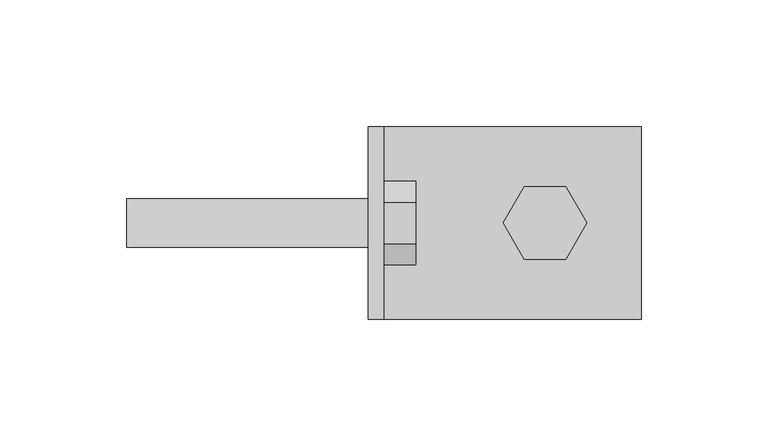
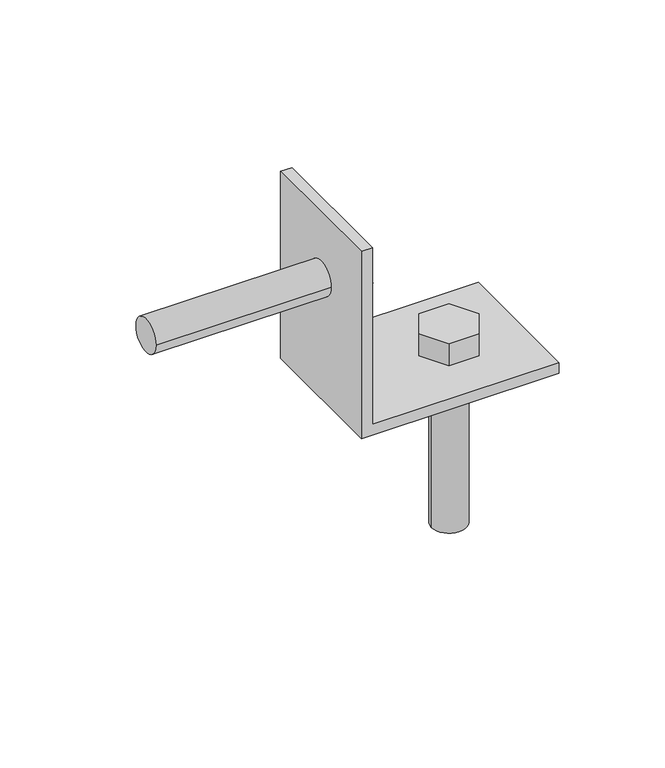
"""IFC4 building model written with IfcOpenShell, lengths in millimetres: fastener geometry, SIMPSON - HLPC/HLGPC Heavy Angles and Gussets : SIMPSON - HL43 - 3 X 4.25 - .75 Bolt - HDG."""

import ifcopenshell
import ifcopenshell.guid

model = None  # the IFC model being written
_history = None  # IfcOwnerHistory: only IFC2X3 demands one
_inside = {}  # id of a spatial element -> (the spatial element, [elements in it])
_under = {}  # id of a project, library or spatial element -> (it, [spatial elements below it])
_declared = {}  # id of a project -> (the project, [libraries it declares])
_typed = {}  # id of a type object -> (the type object, [elements of that type])
_made_of = {}  # id of a material, layer set ... -> (it, [elements and type objects made of it])


def new_model(schema):
    """Start an empty IFC model of exactly this schema.

    Asked for "IFC4X3", IfcOpenShell would pick the latest addendum, in which some entities
    have other attributes; the version numbers below select the first issue.
    IFC2X3 requires an IfcOwnerHistory on every rooted entity: one is made here for all.
    """
    global model, _history
    if schema == "IFC4X3":
        model = ifcopenshell.file(schema_version=(4, 3, 0, 0))
    else:
        model = ifcopenshell.file(schema=schema)
    _inside.clear()
    _under.clear()
    _declared.clear()
    _typed.clear()
    _made_of.clear()
    _history = None
    if model.schema == "IFC2X3":
        org = make("IfcOrganization", Name="unknown")
        user = make(
            "IfcPersonAndOrganization",
            ThePerson=make("IfcPerson", FamilyName="unknown"),
            TheOrganization=org,
        )
        app = make(
            "IfcApplication",
            ApplicationDeveloper=org,
            Version="unknown",
            ApplicationFullName="unknown",
            ApplicationIdentifier="unknown",
        )
        _history = make(
            "IfcOwnerHistory",
            OwningUser=user,
            OwningApplication=app,
            ChangeAction="ADDED",
            CreationDate=0,
        )
    return model


def make(cls, **values):
    """One entity of the class cls with the attributes given. An attribute that is None is left unset."""
    return model.create_entity(
        cls, **{name: value for name, value in values.items() if value is not None}
    )


def rooted(cls, **values):
    """An entity with a GlobalId (a new one), such as an element, a storey or a relation."""
    return make(cls, GlobalId=ifcopenshell.guid.new(), OwnerHistory=_history, **values)


def si_unit(unit_type, name, prefix=None):
    """IfcSIUnit, for example si_unit("LENGTHUNIT", "METRE", prefix="MILLI")."""
    return make("IfcSIUnit", UnitType=unit_type, Prefix=prefix, Name=name)


def assignment(units):
    """IfcUnitAssignment: the units of a project."""
    return None if units is None else make("IfcUnitAssignment", Units=units)


def point(xyz):
    """IfcCartesianPoint."""
    return None if xyz is None else make("IfcCartesianPoint", Coordinates=xyz)


def direction(xyz):
    """IfcDirection."""
    return None if xyz is None else make("IfcDirection", DirectionRatios=xyz)


def frame(location, z_axis=None, x_axis=None):
    """IfcAxis2Placement3D, a coordinate frame: its origin and axes. An axis left out is left unset."""
    return make(
        "IfcAxis2Placement3D",
        Location=point(location),
        Axis=direction(z_axis),
        RefDirection=direction(x_axis),
    )


def frame_2d(location, x_axis=None):
    """IfcAxis2Placement2D, a coordinate frame in the plane: its origin and x axis."""
    return make(
        "IfcAxis2Placement2D", Location=point(location), RefDirection=direction(x_axis)
    )


def origin():
    """The frame at (0, 0, 0) with its axes left unset."""
    return frame((0.0, 0.0, 0.0))


def place(relative_to, where):
    """IfcLocalPlacement: puts the frame where relative to a parent placement (None: the world)."""
    return make(
        "IfcLocalPlacement", PlacementRelTo=relative_to, RelativePlacement=where
    )


def context(
    kind, dimensions, precision=None, world=None, true_north=None, identifier=None
):
    """IfcGeometricRepresentationContext, for example the 3D "Model" context."""
    return make(
        "IfcGeometricRepresentationContext",
        ContextIdentifier=identifier,
        ContextType=kind,
        CoordinateSpaceDimension=dimensions,
        Precision=precision,
        WorldCoordinateSystem=world,
        TrueNorth=true_north,
    )


def project(units=None, contexts=None):
    """IfcProject with its units and contexts."""
    return rooted(
        "IfcProject",
        Name="project",
        RepresentationContexts=contexts,
        UnitsInContext=assignment(units),
    )


def spatial(cls, under=None, at=None, **own):
    """A site, building, storey or space (cls), placed at a placement, below another one or the project."""
    s = rooted(cls, ObjectPlacement=at, **own)
    if under is not None:
        _under.setdefault(under.id(), (under, []))[1].append(s)
    return s


def polyline(points):
    """IfcPolyline through the points."""
    return make("IfcPolyline", Points=[point(p) for p in points])


def circle_curve(where, radius):
    """IfcCircle in the frame where."""
    return make("IfcCircle", Position=where, Radius=radius)


def trimmed(basis, trim1, trim2, sense, master):
    """IfcTrimmedCurve: the piece of a basis curve between two trims."""
    return make(
        "IfcTrimmedCurve",
        BasisCurve=basis,
        Trim1=trim1,
        Trim2=trim2,
        SenseAgreement=sense,
        MasterRepresentation=master,
    )


def segment(curve, same_sense, transition):
    """IfcCompositeCurveSegment."""
    return make(
        "IfcCompositeCurveSegment",
        Transition=transition,
        SameSense=same_sense,
        ParentCurve=curve,
    )


def composite_curve(segments, self_intersect=None):
    """IfcCompositeCurve: segments joined end to end."""
    return make("IfcCompositeCurve", Segments=segments, SelfIntersect=self_intersect)


def outline(outer, holes=None, kind="AREA"):
    """IfcArbitraryClosedProfileDef: a profile drawn as a closed curve; with holes, ...WithVoids."""
    if holes is None:
        return make("IfcArbitraryClosedProfileDef", ProfileType=kind, OuterCurve=outer)
    return make(
        "IfcArbitraryProfileDefWithVoids",
        ProfileType=kind,
        OuterCurve=outer,
        InnerCurves=holes,
    )


def extrude(swept, where, along, depth):
    """IfcExtrudedAreaSolid: the profile swept, set in the frame where, extruded along a direction by depth."""
    return make(
        "IfcExtrudedAreaSolid",
        SweptArea=swept,
        Position=where,
        ExtrudedDirection=direction(along),
        Depth=depth,
    )


def shape(context_of_items, identifier, shape_type, items):
    """IfcShapeRepresentation: the items that make up one representation, for example the "Body"."""
    return make(
        "IfcShapeRepresentation",
        ContextOfItems=context_of_items,
        RepresentationIdentifier=identifier,
        RepresentationType=shape_type,
        Items=items,
    )


def source(mapping_origin, context_of_items, identifier, shape_type, items):
    """IfcRepresentationMap: a shape defined once, which mapped items show again and again."""
    return make(
        "IfcRepresentationMap",
        MappingOrigin=mapping_origin,
        MappedRepresentation=shape(context_of_items, identifier, shape_type, items),
    )


def transform(
    local_origin,
    x_axis=None,
    y_axis=None,
    z_axis=None,
    scale=None,
    scale2=None,
    scale3=None,
    uniform=True,
):
    """IfcCartesianTransformationOperator3D, or its non-uniform kind. x_axis, y_axis, z_axis: its Axis1, 2, 3."""
    if uniform:
        return make(
            "IfcCartesianTransformationOperator3D",
            Axis1=direction(x_axis),
            Axis2=direction(y_axis),
            LocalOrigin=point(local_origin),
            Scale=scale,
            Axis3=direction(z_axis),
        )
    return make(
        "IfcCartesianTransformationOperator3DnonUniform",
        Axis1=direction(x_axis),
        Axis2=direction(y_axis),
        LocalOrigin=point(local_origin),
        Scale=scale,
        Axis3=direction(z_axis),
        Scale2=scale2,
        Scale3=scale3,
    )


def mapped(mapping_source, mapping_target):
    """IfcMappedItem: shows the shape of a source again, moved by a transform."""
    return make(
        "IfcMappedItem", MappingSource=mapping_source, MappingTarget=mapping_target
    )


def made_of(thing, what):
    """Note that an element or type object is made of a material, layer set ...; save() writes the relation."""
    if what is not None:
        _made_of.setdefault(what.id(), (what, []))[1].append(thing)
    return thing


def element(
    cls,
    number,
    at=None,
    inside=None,
    cuts=None,
    type_object=None,
    material=None,
    context=None,
    identifier="Body",
    shape_type=None,
    held_by="IfcProductDefinitionShape",
    body=None,
    shapes=None,
    **own,
):
    """One element of the class cls, such as IfcWall. Its Tag is "e" and its number.

    at: its placement. inside: the storey or other place that contains it. cuts: it is an
    opening in that element (IfcRelVoidsElement). A single representation is given by context,
    identifier, shape_type and body (its items); several are given by shapes. held_by: the class
    of the entity that holds the representations. save() writes the other relations.
    """
    e = rooted(cls, Tag="e%d" % number, ObjectPlacement=at, **own)
    if body is not None:
        shapes = [shape(context, identifier, shape_type, body)]
    if shapes is not None:
        e.Representation = make(held_by, Representations=shapes)
    if inside is not None:
        _inside.setdefault(inside.id(), (inside, []))[1].append(e)
    if cuts is not None:
        rooted(
            "IfcRelVoidsElement", RelatingBuildingElement=cuts, RelatedOpeningElement=e
        )
    if type_object is not None:
        _typed.setdefault(type_object.id(), (type_object, []))[1].append(e)
    return made_of(e, material)


def aggregate(whole, parts):
    """IfcRelAggregates: a whole, such as a stair, and the parts it consists of."""
    return rooted("IfcRelAggregates", RelatingObject=whole, RelatedObjects=parts)


def save(model, path):
    """Write the relations noted so far, then the file.

    IfcRelAggregates (storeys below a building ...), IfcRelContainedInSpatialStructure (elements
    in a storey), IfcRelDefinesByType, IfcRelAssociatesMaterial and IfcRelDeclares: one each for
    every whole, place, type object, material and project.
    """
    for whole, parts in _under.values():
        aggregate(whole, parts)
    for where, things in _inside.values():
        rooted(
            "IfcRelContainedInSpatialStructure",
            RelatedElements=things,
            RelatingStructure=where,
        )
    for kind, things in _typed.values():
        rooted("IfcRelDefinesByType", RelatedObjects=things, RelatingType=kind)
    for what, things in _made_of.values():
        rooted("IfcRelAssociatesMaterial", RelatedObjects=things, RelatingMaterial=what)
    for by, libraries in _declared.values():
        rooted("IfcRelDeclares", RelatingContext=by, RelatedDefinitions=libraries)
    model.write(path)


def plane_surface(at):
    """IfcPlane: the flat surface through the origin of the frame at, square to its z axis."""
    return make("IfcPlane", Position=at)


def revolved_surface(curve, axis_point, axis_direction):
    """IfcSurfaceOfRevolution: the curve turned about the line through axis_point along axis_direction."""
    return make(
        "IfcSurfaceOfRevolution",
        SweptCurve=make("IfcArbitraryOpenProfileDef", ProfileType="CURVE", Curve=curve),
        AxisPosition=make("IfcAxis1Placement", Location=point(axis_point), Axis=direction(axis_direction)),
    )


def advanced_brep(points, edges, surfaces, faces):
    """IfcAdvancedBrep: a solid bounded by faces that lie on surfaces and meet in shared edges.

    An edge is (start, end): straight between two places in points (the first is 0);
    or (start, end, curve); or (start, end, curve, False) where it runs against its curve.
    A face is (place in surfaces, loops), or (place, loops, False) where it looks against
    its surface's normal. A loop lists edges by number (the first is 1), with a minus sign
    where the edge is run from its end to its start. The first loop is the outer one.
    """
    corners = [point(p) for p in points]
    vertices = [make("IfcVertexPoint", VertexGeometry=c) for c in corners]
    made = []
    for start, end, *more in edges:
        made.append(
            make(
                "IfcEdgeCurve",
                EdgeStart=vertices[start],
                EdgeEnd=vertices[end],
                EdgeGeometry=more[0] if more else make("IfcPolyline", Points=[corners[start], corners[end]]),
                SameSense=more[1] if len(more) > 1 else True,
            )
        )
    hull = []
    for where, loops, *sense in faces:
        bounds = []
        for j, loop in enumerate(loops):
            ring = [make("IfcOrientedEdge", EdgeElement=made[abs(k) - 1], Orientation=k > 0) for k in loop]
            bounds.append(
                make(
                    "IfcFaceOuterBound" if j == 0 else "IfcFaceBound",
                    Bound=make("IfcEdgeLoop", EdgeList=ring),
                    Orientation=True,
                )
            )
        hull.append(make("IfcAdvancedFace", Bounds=bounds, FaceSurface=surfaces[where], SameSense=sense[0] if sense else True))
    return make("IfcAdvancedBrep", Outer=make("IfcClosedShell", CfsFaces=hull))


def fastener_c5b4ea8f(model_context):
    return source(origin(), model_context, "Body", "SolidModel", [
        extrude(outline(composite_curve([segment(trimmed(circle_curve(frame_2d((0.0, 69.85)), 9.525), [point((-9.525, 69.85))], [point((9.525, 69.85))], False, "CARTESIAN"), True, "CONTINUOUS"), segment(trimmed(circle_curve(frame_2d((0.0, 69.85)), 9.525), [point((9.525, 69.85))], [point((-9.525, 69.85))], False, "CARTESIAN"), True, "CONTINUOUS")], self_intersect=False)), frame((-95.5476562, 0.0, 0.0), z_axis=(1.0, 0.0, 0.0), x_axis=(0.0, 1.0, 0.0)), (0.0, 0.0, 1.0), 101.6),
        extrude(outline(polyline([(-16.4977839, 69.85), (-8.248892, 84.1375), (8.248892, 84.1375), (16.4977839, 69.85), (8.248892, 55.5625), (-8.248892, 55.5625), (-16.4977839, 69.85)])), frame((6.0523438, 0.0, 0.0), z_axis=(1.0, 0.0, 0.0), x_axis=(0.0, 1.0, 0.0)), (0.0, 0.0, 1.0), 12.7),
        extrude(outline(composite_curve([segment(trimmed(circle_curve(frame_2d((69.85, 0.0)), 9.525), [point((60.325, 0.0))], [point((79.375, 0.0))], False, "CARTESIAN"), True, "CONTINUOUS"), segment(trimmed(circle_curve(frame_2d((69.85, 0.0)), 9.525), [point((79.375, 0.0))], [point((60.325, 0.0))], False, "CARTESIAN"), True, "CONTINUOUS")], self_intersect=False)), frame((0.0, 0.0, -95.5476563), z_axis=(0.0, 0.0, 1.0), x_axis=(1.0, 0.0, 0.0)), (0.0, 0.0, 1.0), 101.6),
        extrude(outline(polyline([(53.3522161, 0.0), (61.601108, 14.2875), (78.098892, 14.2875), (86.3477839, 0.0), (78.098892, -14.2875), (61.601108, -14.2875), (53.3522161, 0.0)])), frame((0.0, 0.0, 6.0523437), z_axis=(0.0, 0.0, 1.0), x_axis=(1.0, 0.0, 0.0)), (0.0, 0.0, 1.0), 12.7),
        advanced_brep(
        [(6.0523438, 38.1, 107.95), (6.0523438, -38.1, 107.95), (6.0523438, -38.1, 6.0523437), (6.0523438, 38.1, 6.0523437), (6.0523438, 9.525, 69.85), (6.0523438, -9.525, 69.85), (0.0, -38.1, 107.95), (0.0, 38.1, 107.95), (0.0, 38.1, 0.0), (0.0, -38.1, 0.0), (0.0, -9.525, 69.85), (0.0, 9.525, 69.85), (107.95, -38.1, 0.0), (107.95, -38.1, 6.0523437), (107.95, 38.1, 6.0523437), (107.95, 38.1, 0.0), (79.375, 0.0, 6.0523437), (60.325, 0.0, 6.0523437), (60.325, 0.0, 0.0), (79.375, 0.0, 0.0)],
        [
            (0, 1),
            (1, 2),
            (2, 3),
            (3, 0),
            (4, 5, circle_curve(frame((6.0523438, 0.0, 69.85), z_axis=(-1.0, 0.0, 0.0), x_axis=(0.0, 1.0, 0.0)), 9.525)),
            (5, 4, circle_curve(frame((6.0523438, 0.0, 69.85), z_axis=(-1.0, 0.0, 0.0), x_axis=(0.0, 1.0, 0.0)), 9.525)),
            (6, 7),
            (7, 8),
            (8, 9),
            (9, 6),
            (10, 11, circle_curve(frame((0.0, 0.0, 69.85), z_axis=(1.0, 0.0, 0.0), x_axis=(0.0, 1.0, 0.0)), 9.525)),
            (11, 10, circle_curve(frame((0.0, 0.0, 69.85), z_axis=(1.0, 0.0, 0.0), x_axis=(0.0, 1.0, 0.0)), 9.525)),
            (0, 7),
            (6, 1),
            (9, 12),
            (12, 13),
            (13, 2),
            (3, 14),
            (14, 15),
            (15, 8),
            (13, 14),
            (16, 17, circle_curve(frame((69.85, 0.0, 6.0523437), z_axis=(0.0, 0.0, -1.0), x_axis=(1.0, 0.0, 0.0)), 9.525)),
            (17, 16, circle_curve(frame((69.85, 0.0, 6.0523437), z_axis=(0.0, 0.0, -1.0), x_axis=(1.0, 0.0, 0.0)), 9.525)),
            (15, 12),
            (18, 19, circle_curve(frame((69.85, 0.0, 0.0), z_axis=(0.0, 0.0, 1.0), x_axis=(1.0, 0.0, 0.0)), 9.525)),
            (19, 18, circle_curve(frame((69.85, 0.0, 0.0), z_axis=(0.0, 0.0, 1.0), x_axis=(1.0, 0.0, 0.0)), 9.525)),
            (16, 19),
            (18, 17),
            (4, 11),
            (10, 5),
        ],
        [
            plane_surface(frame((6.0523438, -38.1, 107.95), z_axis=(1.0, 0.0, 0.0), x_axis=(0.0, -1.0, 0.0))),
            plane_surface(frame((0.0, -38.1, 107.95), z_axis=(-1.0, 0.0, 0.0), x_axis=(0.0, 1.0, 0.0))),
            plane_surface(frame((6.0523438, 38.1, 107.95), z_axis=(0.0, 0.0, 1.0), x_axis=(-1.0, 0.0, 0.0))),
            plane_surface(frame((6.0523438, -38.1, 107.95), z_axis=(0.0, -1.0, 0.0), x_axis=(-1.0, 0.0, 0.0))),
            plane_surface(frame((6.0523438, 38.1, 6.0523437), z_axis=(0.0, 1.0, 0.0), x_axis=(-1.0, 0.0, 0.0))),
            plane_surface(frame((0.0, 38.1, 6.0523437), z_axis=(0.0, 0.0, 1.0), x_axis=(-1.0, 0.0, 0.0))),
            plane_surface(frame((0.0, 38.1, 0.0), z_axis=(0.0, 0.0, -1.0), x_axis=(1.0, 0.0, 0.0))),
            plane_surface(frame((107.95, -38.1, 6.0523437), z_axis=(1.0, 0.0, 0.0), x_axis=(0.0, 0.0, -1.0))),
            revolved_surface(polyline([(79.375, 0.0, 6.0523437), (79.375, 0.0, 0.0)]), (69.85, 0.0, 0.0), (0.0, 0.0, 1.0)),
            revolved_surface(polyline([(6.0523438, 9.525, 69.85), (0.0, 9.525, 69.85)]), (0.0, 0.0, 69.85), (1.0, 0.0, 0.0)),
        ],
        [
            (0, [[1, 2, 3, 4], [5, 6]]),
            (1, [[7, 8, 9, 10], [11, 12]]),
            (2, [[-1, 13, -7, 14]]),
            (3, [[-2, -14, -10, 15, 16, 17]]),
            (4, [[-4, 18, 19, 20, -8, -13]]),
            (5, [[21, -18, -3, -17], [22, 23]]),
            (6, [[24, -15, -9, -20], [25, 26]]),
            (7, [[-21, -16, -24, -19]]),
            (8, [[27, -25, 28, -22]]),
            (8, [[-27, -23, -28, -26]]),
            (9, [[29, -11, 30, -5]]),
            (9, [[-29, -6, -30, -12]]),
        ],
    ),
    ])


if __name__ == "__main__":
    model = new_model("IFC4")
    model_context = context("Model", 3, world=origin())
    ifc_project = project(units=[si_unit("LENGTHUNIT", "METRE", prefix="MILLI")], contexts=[model_context])
    site = spatial("IfcSite", under=ifc_project)
    building = spatial("IfcBuilding", under=site)
    placement = place(None, origin())
    fastener_shape = fastener_c5b4ea8f(model_context)
    element("IfcFastener", 1, ObjectType="SIMPSON - HLPC/HLGPC Heavy Angles and Gussets : SIMPSON - HL43 - 3 X 4.25 - .75 Bolt - HDG", at=placement, inside=building, context=model_context, shape_type="MappedRepresentation", body=[
        mapped(fastener_shape, transform((0.0, 0.0, 0.0), x_axis=(1.0, 0.0, 0.0), y_axis=(0.0, 1.0, 0.0), z_axis=(0.0, 0.0, 1.0))),
    ])
    save(model, "model.ifc")

# Revit data of these elements
# Type "SIMPSON - HLPC/HLGPC Heavy Angles and Gussets : SIMPSON - HL43 - 3 X 4.25 - .75 Bolt - HDG"
#   URL = "https://www.strongtie.com/classiccollection_architecturalproductsgroup/hlpc-hlgpc_productgroup_wcc/p/hlpc.hlgpc"
#   L = 0' - 3"
#   Hole Radius = 0' - 0 3/8"
#   D4 = 0' - 5"
#   D2 = 0' - 5"
#   D1 = 0' - 1 1/2"
#   D3 = 0' - 2 3/4"
#   Ga. = 0' - 0 61/256"
#   W1 & W2 = 0' - 4 1/4"
#   Default Elevation = 4' - 0"
#   Bolt Visibility - 3B = no
#   Bolt Visibility - 3A = no
#   Bolt Visibility - 2B = no
#   Bolt Visibility - 2A = no
#   Bolt Visibility - 1B = no
#   Bolt Visibility - 1A = yes
#   Bolt Visibility = yes
#   Bolt Size = element 1298415
# Element 1 (IfcFastener, "SIMPSON - HLPC/HLGPC Heavy Angles and Gussets : SIMPSON - HL43 - 3 X 4.25 - .75 Bolt - HDG")
#   Materials on its faces: "1\" GALV. LAG BOLT (LENGTH = 1/2\" SHY OF GLULAM DEPTH) -  (GALV. THRU BOLT IF PLATE ON OPP. SIDE OF STRUCT MEMBER)"
# Materials
#   "1\" GALV. LAG BOLT (LENGTH = 1/2\" SHY OF GLULAM DEPTH) -  (GALV. THRU BOLT IF PLATE ON OPP. SIDE OF STRUCT MEMBER)": class "Generic", colour RGB 120 120 120, transparency 0, Cost = 0
